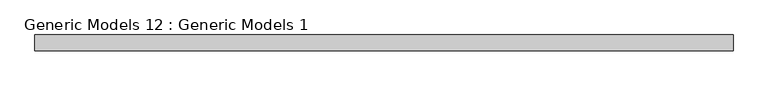
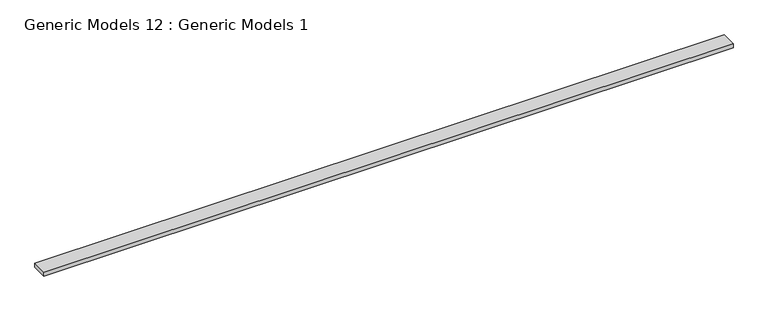
"""IFC4 building model written with IfcOpenShell, lengths in millimetres: proxy geometry, Generic Models 12 : Generic Models 1."""

from ifc_helpers import new_model, si_unit, frame, origin, place, context, project, spatial, polyline, outline, extrude, source, transform, mapped, element, save


def generic_models_12_generic_models_1_3ee93f90(model_context):
    return source(origin(), model_context, "Body", "SweptSolid", [
        extrude(outline(polyline([(2196.9263704, -7055.4230338), (2196.9263704, -6915.7230338), (8386.8578684, -6915.7230338), (8386.8578684, -7055.4230338), (2196.9263704, -7055.4230338)])), frame((0.0, 0.0, 126783.846), z_axis=(0.0, 0.0, 1.0), x_axis=(1.0, 0.0, 0.0)), (0.0, 0.0, 1.0), 38.1),
    ])


if __name__ == "__main__":
    model = new_model("IFC4")
    model_context = context("Model", 3, world=origin())
    ifc_project = project(units=[si_unit("LENGTHUNIT", "METRE", prefix="MILLI")], contexts=[model_context])
    site = spatial("IfcSite", under=ifc_project)
    building = spatial("IfcBuilding", under=site)
    placement = place(None, origin())
    generic_models_12_generic_models_1_shape = generic_models_12_generic_models_1_3ee93f90(model_context)
    element("IfcBuildingElementProxy", 1, Name="Generic Models 12 : Generic Models 1", ObjectType="Generic Models 12 : Generic Models 1", at=placement, inside=building, context=model_context, shape_type="MappedRepresentation", body=[
        mapped(generic_models_12_generic_models_1_shape, transform((0.0, 0.0, 0.0), x_axis=(1.0, 0.0, 0.0), y_axis=(0.0, 1.0, 0.0), z_axis=(0.0, 0.0, 1.0))),
    ])
    save(model, "model.ifc")

# Revit data of these elements
# Element 1 (IfcBuildingElementProxy, "Generic Models 12 : Generic Models 1")
#   Materials on its faces: "_2X BLOCKING AS REQUIRED"
# Materials
#   "_2X BLOCKING AS REQUIRED": class "Generic", colour RGB 177 130 114, transparency 0, Cost = 0
